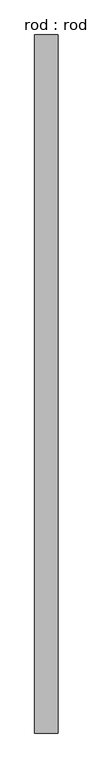
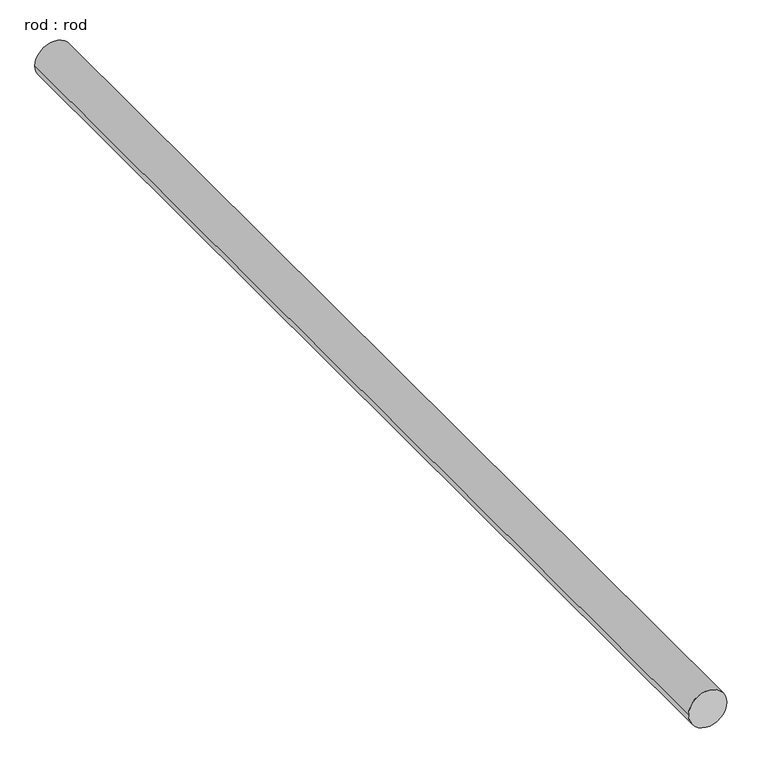
"""IFC4 building model written with IfcOpenShell, lengths in millimetres: proxy geometry, rod : rod."""

from ifc_helpers import new_model, si_unit, point, frame, frame_2d, origin, place, context, project, spatial, circle_curve, trimmed, segment, composite_curve, outline, extrude, source, transform, mapped, element, save


def rod_rod_5cf49b49(model_context):
    return source(origin(), model_context, "Body", "SweptSolid", [
        extrude(outline(composite_curve([segment(trimmed(circle_curve(frame_2d((0.0108462, 0.0)), 200.0), [point((0.0108462, 200.0))], [point((0.0108462, -200.0))], False, "CARTESIAN"), True, "CONTINUOUS"), segment(trimmed(circle_curve(frame_2d((0.0108462, 0.0)), 200.0), [point((0.0108462, -200.0))], [point((0.0108462, 200.0))], False, "CARTESIAN"), True, "CONTINUOUS")], self_intersect=False)), frame((0.0, -1830.8872742, 0.0), z_axis=(0.0, 1.0, 0.0), x_axis=(0.0, 0.0, 1.0)), (0.0, 0.0, 1.0), 11847.231779),
    ])


if __name__ == "__main__":
    model = new_model("IFC4")
    model_context = context("Model", 3, world=origin())
    ifc_project = project(units=[si_unit("LENGTHUNIT", "METRE", prefix="MILLI")], contexts=[model_context])
    site = spatial("IfcSite", under=ifc_project)
    building = spatial("IfcBuilding", under=site)
    placement = place(None, origin())
    rod_rod_shape = rod_rod_5cf49b49(model_context)
    element("IfcBuildingElementProxy", 1, Name="rod : rod", ObjectType="rod : rod", at=placement, inside=building, context=model_context, shape_type="MappedRepresentation", body=[
        mapped(rod_rod_shape, transform((0.0, 0.0, 0.0), x_axis=(1.0, 0.0, 0.0), y_axis=(0.0, 1.0, 0.0), z_axis=(0.0, 0.0, 1.0))),
    ])
    save(model, "model.ifc")

# Revit data of these elements
# Type "rod : rod"
#   Default Elevation = 0
